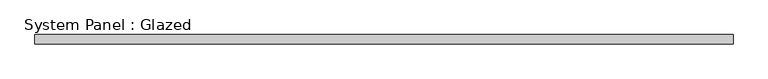
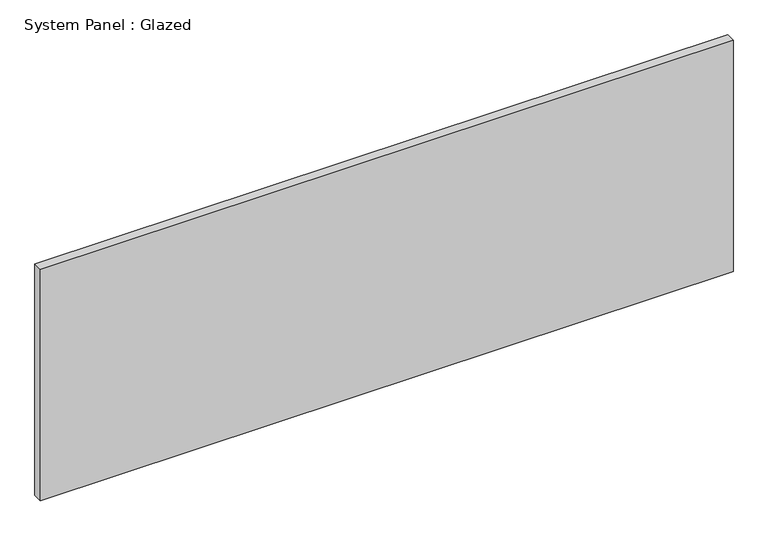
"""IFC4 building model written with IfcOpenShell, lengths in millimetres: plate geometry, System Panel : Glazed."""

from ifc_helpers import new_model, si_unit, origin, origin_with_axes, place, context, project, spatial, polyline, outline, extrude, source, transform, mapped, element, save


def system_panel_glazed_c322100e(model_context):
    return source(origin(), model_context, "Body", "SweptSolid", [
        extrude(outline(polyline([(919.4444444, 24.5), (-919.4444444, 24.5), (-919.4444444, 49.5), (919.4444444, 49.5), (919.4444444, 24.5)])), origin_with_axes(), (0.0, 0.0, 1.0), 650.0),
    ])


if __name__ == "__main__":
    model = new_model("IFC4")
    model_context = context("Model", 3, world=origin())
    ifc_project = project(units=[si_unit("LENGTHUNIT", "METRE", prefix="MILLI")], contexts=[model_context])
    site = spatial("IfcSite", under=ifc_project)
    building = spatial("IfcBuilding", under=site)
    placement = place(None, origin())
    system_panel_glazed_shape = system_panel_glazed_c322100e(model_context)
    element("IfcPlate", 1, ObjectType="System Panel : Glazed", at=placement, inside=building, context=model_context, shape_type="MappedRepresentation", body=[
        mapped(system_panel_glazed_shape, transform((0.0, 0.0, 0.0), x_axis=(1.0, 0.0, 0.0), y_axis=(0.0, 1.0, 0.0), z_axis=(0.0, 0.0, 1.0))),
    ])
    save(model, "model.ifc")

# Revit data of these elements
# Element 1 (IfcPlate, "System Panel : Glazed")
#   Materials on its faces: "Glass"
# Materials
#   "Glass": class "Glass", colour RGB 0 128 192, transparency 0.9
